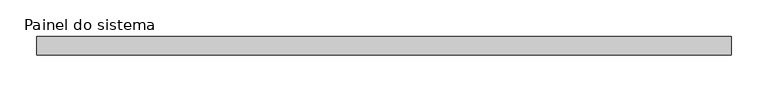
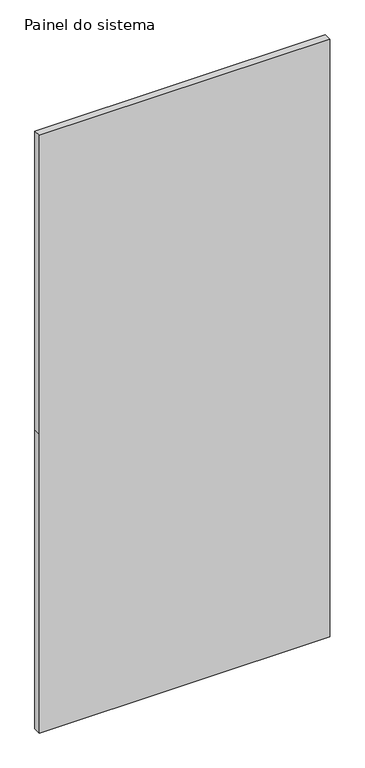
"""IFC4 building model written with IfcOpenShell, lengths in millimetres: plate geometry, Painel do sistema : Envidraçado."""

import ifcopenshell
import ifcopenshell.guid

model = None  # the IFC model being written
_history = None  # IfcOwnerHistory: only IFC2X3 demands one
_inside = {}  # id of a spatial element -> (the spatial element, [elements in it])
_under = {}  # id of a project, library or spatial element -> (it, [spatial elements below it])
_declared = {}  # id of a project -> (the project, [libraries it declares])
_typed = {}  # id of a type object -> (the type object, [elements of that type])
_made_of = {}  # id of a material, layer set ... -> (it, [elements and type objects made of it])


def new_model(schema):
    """Start an empty IFC model of exactly this schema.

    Asked for "IFC4X3", IfcOpenShell would pick the latest addendum, in which some entities
    have other attributes; the version numbers below select the first issue.
    IFC2X3 requires an IfcOwnerHistory on every rooted entity: one is made here for all.
    """
    global model, _history
    if schema == "IFC4X3":
        model = ifcopenshell.file(schema_version=(4, 3, 0, 0))
    else:
        model = ifcopenshell.file(schema=schema)
    _inside.clear()
    _under.clear()
    _declared.clear()
    _typed.clear()
    _made_of.clear()
    _history = None
    if model.schema == "IFC2X3":
        org = make("IfcOrganization", Name="unknown")
        user = make(
            "IfcPersonAndOrganization",
            ThePerson=make("IfcPerson", FamilyName="unknown"),
            TheOrganization=org,
        )
        app = make(
            "IfcApplication",
            ApplicationDeveloper=org,
            Version="unknown",
            ApplicationFullName="unknown",
            ApplicationIdentifier="unknown",
        )
        _history = make(
            "IfcOwnerHistory",
            OwningUser=user,
            OwningApplication=app,
            ChangeAction="ADDED",
            CreationDate=0,
        )
    return model


def make(cls, **values):
    """One entity of the class cls with the attributes given. An attribute that is None is left unset."""
    return model.create_entity(
        cls, **{name: value for name, value in values.items() if value is not None}
    )


def rooted(cls, **values):
    """An entity with a GlobalId (a new one), such as an element, a storey or a relation."""
    return make(cls, GlobalId=ifcopenshell.guid.new(), OwnerHistory=_history, **values)


def si_unit(unit_type, name, prefix=None):
    """IfcSIUnit, for example si_unit("LENGTHUNIT", "METRE", prefix="MILLI")."""
    return make("IfcSIUnit", UnitType=unit_type, Prefix=prefix, Name=name)


def assignment(units):
    """IfcUnitAssignment: the units of a project."""
    return None if units is None else make("IfcUnitAssignment", Units=units)


def point(xyz):
    """IfcCartesianPoint."""
    return None if xyz is None else make("IfcCartesianPoint", Coordinates=xyz)


def direction(xyz):
    """IfcDirection."""
    return None if xyz is None else make("IfcDirection", DirectionRatios=xyz)


def frame(location, z_axis=None, x_axis=None):
    """IfcAxis2Placement3D, a coordinate frame: its origin and axes. An axis left out is left unset."""
    return make(
        "IfcAxis2Placement3D",
        Location=point(location),
        Axis=direction(z_axis),
        RefDirection=direction(x_axis),
    )


def origin():
    """The frame at (0, 0, 0) with its axes left unset."""
    return frame((0.0, 0.0, 0.0))


def place(relative_to, where):
    """IfcLocalPlacement: puts the frame where relative to a parent placement (None: the world)."""
    return make(
        "IfcLocalPlacement", PlacementRelTo=relative_to, RelativePlacement=where
    )


def context(
    kind, dimensions, precision=None, world=None, true_north=None, identifier=None
):
    """IfcGeometricRepresentationContext, for example the 3D "Model" context."""
    return make(
        "IfcGeometricRepresentationContext",
        ContextIdentifier=identifier,
        ContextType=kind,
        CoordinateSpaceDimension=dimensions,
        Precision=precision,
        WorldCoordinateSystem=world,
        TrueNorth=true_north,
    )


def project(units=None, contexts=None):
    """IfcProject with its units and contexts."""
    return rooted(
        "IfcProject",
        Name="project",
        RepresentationContexts=contexts,
        UnitsInContext=assignment(units),
    )


def spatial(cls, under=None, at=None, **own):
    """A site, building, storey or space (cls), placed at a placement, below another one or the project."""
    s = rooted(cls, ObjectPlacement=at, **own)
    if under is not None:
        _under.setdefault(under.id(), (under, []))[1].append(s)
    return s


def polyline(points):
    """IfcPolyline through the points."""
    return make("IfcPolyline", Points=[point(p) for p in points])


def outline(outer, holes=None, kind="AREA"):
    """IfcArbitraryClosedProfileDef: a profile drawn as a closed curve; with holes, ...WithVoids."""
    if holes is None:
        return make("IfcArbitraryClosedProfileDef", ProfileType=kind, OuterCurve=outer)
    return make(
        "IfcArbitraryProfileDefWithVoids",
        ProfileType=kind,
        OuterCurve=outer,
        InnerCurves=holes,
    )


def extrude(swept, where, along, depth):
    """IfcExtrudedAreaSolid: the profile swept, set in the frame where, extruded along a direction by depth."""
    return make(
        "IfcExtrudedAreaSolid",
        SweptArea=swept,
        Position=where,
        ExtrudedDirection=direction(along),
        Depth=depth,
    )


def shape(context_of_items, identifier, shape_type, items):
    """IfcShapeRepresentation: the items that make up one representation, for example the "Body"."""
    return make(
        "IfcShapeRepresentation",
        ContextOfItems=context_of_items,
        RepresentationIdentifier=identifier,
        RepresentationType=shape_type,
        Items=items,
    )


def source(mapping_origin, context_of_items, identifier, shape_type, items):
    """IfcRepresentationMap: a shape defined once, which mapped items show again and again."""
    return make(
        "IfcRepresentationMap",
        MappingOrigin=mapping_origin,
        MappedRepresentation=shape(context_of_items, identifier, shape_type, items),
    )


def transform(
    local_origin,
    x_axis=None,
    y_axis=None,
    z_axis=None,
    scale=None,
    scale2=None,
    scale3=None,
    uniform=True,
):
    """IfcCartesianTransformationOperator3D, or its non-uniform kind. x_axis, y_axis, z_axis: its Axis1, 2, 3."""
    if uniform:
        return make(
            "IfcCartesianTransformationOperator3D",
            Axis1=direction(x_axis),
            Axis2=direction(y_axis),
            LocalOrigin=point(local_origin),
            Scale=scale,
            Axis3=direction(z_axis),
        )
    return make(
        "IfcCartesianTransformationOperator3DnonUniform",
        Axis1=direction(x_axis),
        Axis2=direction(y_axis),
        LocalOrigin=point(local_origin),
        Scale=scale,
        Axis3=direction(z_axis),
        Scale2=scale2,
        Scale3=scale3,
    )


def mapped(mapping_source, mapping_target):
    """IfcMappedItem: shows the shape of a source again, moved by a transform."""
    return make(
        "IfcMappedItem", MappingSource=mapping_source, MappingTarget=mapping_target
    )


def made_of(thing, what):
    """Note that an element or type object is made of a material, layer set ...; save() writes the relation."""
    if what is not None:
        _made_of.setdefault(what.id(), (what, []))[1].append(thing)
    return thing


def element(
    cls,
    number,
    at=None,
    inside=None,
    cuts=None,
    type_object=None,
    material=None,
    context=None,
    identifier="Body",
    shape_type=None,
    held_by="IfcProductDefinitionShape",
    body=None,
    shapes=None,
    **own,
):
    """One element of the class cls, such as IfcWall. Its Tag is "e" and its number.

    at: its placement. inside: the storey or other place that contains it. cuts: it is an
    opening in that element (IfcRelVoidsElement). A single representation is given by context,
    identifier, shape_type and body (its items); several are given by shapes. held_by: the class
    of the entity that holds the representations. save() writes the other relations.
    """
    e = rooted(cls, Tag="e%d" % number, ObjectPlacement=at, **own)
    if body is not None:
        shapes = [shape(context, identifier, shape_type, body)]
    if shapes is not None:
        e.Representation = make(held_by, Representations=shapes)
    if inside is not None:
        _inside.setdefault(inside.id(), (inside, []))[1].append(e)
    if cuts is not None:
        rooted(
            "IfcRelVoidsElement", RelatingBuildingElement=cuts, RelatedOpeningElement=e
        )
    if type_object is not None:
        _typed.setdefault(type_object.id(), (type_object, []))[1].append(e)
    return made_of(e, material)


def aggregate(whole, parts):
    """IfcRelAggregates: a whole, such as a stair, and the parts it consists of."""
    return rooted("IfcRelAggregates", RelatingObject=whole, RelatedObjects=parts)


def save(model, path):
    """Write the relations noted so far, then the file.

    IfcRelAggregates (storeys below a building ...), IfcRelContainedInSpatialStructure (elements
    in a storey), IfcRelDefinesByType, IfcRelAssociatesMaterial and IfcRelDeclares: one each for
    every whole, place, type object, material and project.
    """
    for whole, parts in _under.values():
        aggregate(whole, parts)
    for where, things in _inside.values():
        rooted(
            "IfcRelContainedInSpatialStructure",
            RelatedElements=things,
            RelatingStructure=where,
        )
    for kind, things in _typed.values():
        rooted("IfcRelDefinesByType", RelatedObjects=things, RelatingType=kind)
    for what, things in _made_of.values():
        rooted("IfcRelAssociatesMaterial", RelatedObjects=things, RelatingMaterial=what)
    for by, libraries in _declared.values():
        rooted("IfcRelDeclares", RelatingContext=by, RelatedDefinitions=libraries)
    model.write(path)


def painel_do_sistema_816baa59(model_context):
    return source(origin(), model_context, "Body", "SweptSolid", [
        extrude(outline(polyline([(0.0, -470.855), (0.0, 470.855), (1025.0, 470.855), (2050.0, 470.855), (2050.0, -470.855), (1025.0, -470.855), (0.0, -470.855)])), frame((0.0, -49.5, 0.0), z_axis=(0.0, 1.0, 0.0), x_axis=(0.0, 0.0, 1.0)), (0.0, 0.0, 1.0), 25.0),
    ])


if __name__ == "__main__":
    model = new_model("IFC4")
    model_context = context("Model", 3, world=origin())
    ifc_project = project(units=[si_unit("LENGTHUNIT", "METRE", prefix="MILLI")], contexts=[model_context])
    site = spatial("IfcSite", under=ifc_project)
    building = spatial("IfcBuilding", under=site)
    placement = place(None, origin())
    painel_do_sistema_shape = painel_do_sistema_816baa59(model_context)
    element("IfcPlate", 1, ObjectType="Painel do sistema : Envidraçado", at=placement, inside=building, context=model_context, shape_type="MappedRepresentation", body=[
        mapped(painel_do_sistema_shape, transform((0.0, 0.0, 0.0), x_axis=(1.0, 0.0, 0.0), y_axis=(0.0, 1.0, 0.0), z_axis=(0.0, 0.0, 1.0))),
    ])
    save(model, "model.ifc")

# Revit data of these elements
# Type "Painel do sistema : Envidraçado"
#   Construction Type Id = "GSP4R"
#   Analytic Construction = "Vidraça única Pilkington 1/8 pol"
#   Visual Light Transmittance = 0.9
#   Solar Heat Gain Coefficient = 0.86
#   Heat Transfer Coefficient (U) = 6.7069 W/(m²·K)
# Element 1 (IfcPlate, "Painel do sistema : Envidraçado")
#   Materials on its faces: ".VIDRO GENÉRICO"
# Materials
#   ".VIDRO GENÉRICO": class ".CC_VIDRO", colour RGB 0 128 192, transparency 0.9, Description = "Vidro comum", Cost = 0
